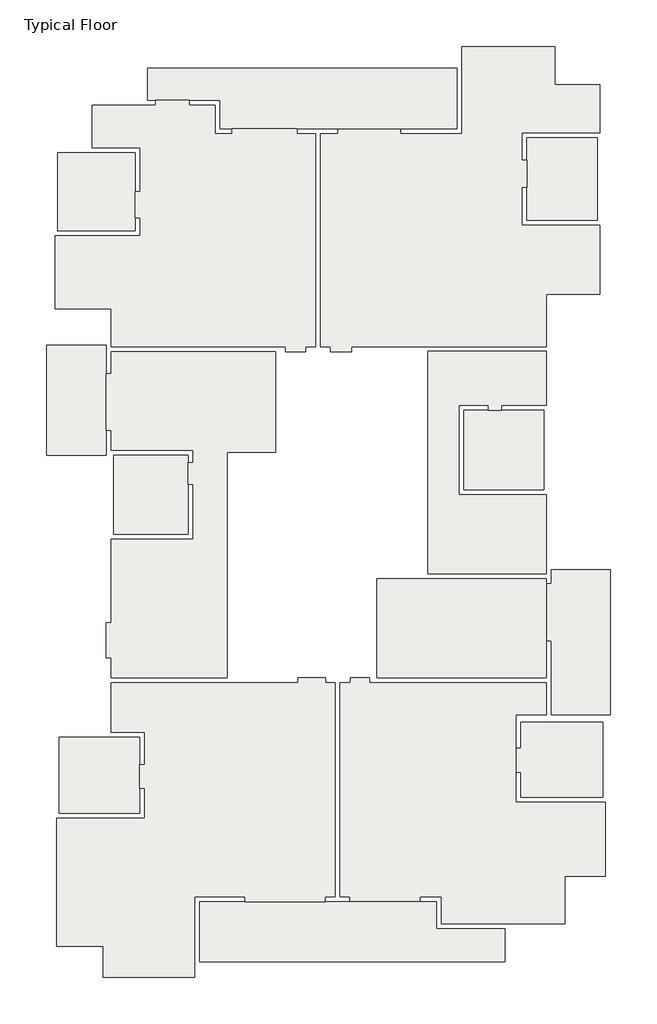
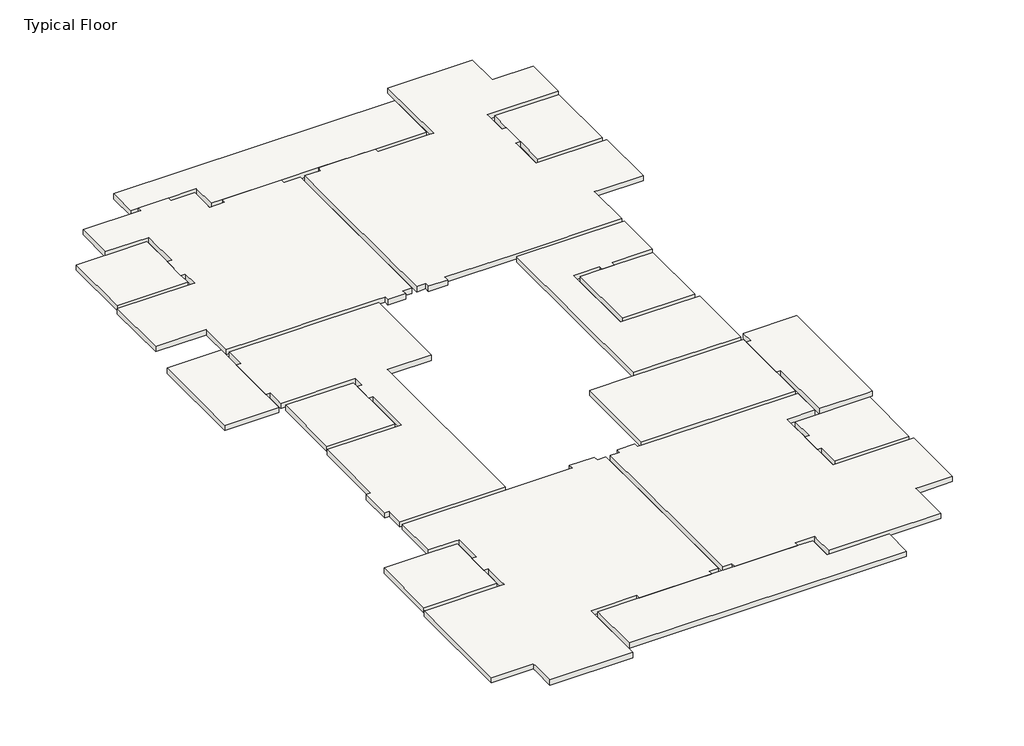
# One storey: 17 slabs.
"""IFC4 building model written with IfcOpenShell, lengths in millimetres."""

from ifc_helpers import new_model, si_unit, frame, origin, place, context, project, spatial, polyline, outline, extrude, faceted_brep, element, save

model = new_model("IFC4")

# Units and contexts
model_context = context("Model", 3, world=origin())
ifc_project = project(units=[si_unit("LENGTHUNIT", "METRE", prefix="MILLI")], contexts=[model_context])

# Site, building, storey
site = spatial("IfcSite", under=ifc_project)
building = spatial("IfcBuilding", under=site)
storey = spatial("IfcBuildingStorey", under=building, Name="Typical Floor", Elevation=3600.0)

# Slabs
placement = place(None, origin())
element("IfcSlab", 1, ObjectType="24", at=placement, inside=storey, context=model_context, shape_type="Brep", body=[
    faceted_brep([(5008.6159742, 7667.3540488, 3360.0), (5008.6159742, 4473.2757833, 3360.0), (1815.6504069, 4473.2757833, 3360.0), (1815.6504069, 7665.1303185, 3360.0), (2790.841428, 7665.1303185, 3360.0), (2790.841428, 7667.3540488, 3360.0), (3310.841428, 7667.3540488, 3360.0), (5008.6159742, 4473.2757833, 3600.0), (5008.6159742, 7667.3540488, 3600.0), (3310.841428, 7667.3540488, 3600.0), (2790.841428, 7667.3540488, 3600.0), (2790.841428, 7665.1303185, 3600.0), (1815.6504069, 7665.1303185, 3600.0), (1815.6504069, 4473.2757833, 3600.0)], [[[0, 1, 2, 3, 4, 5, 6]], [[7, 8, 9, 10, 11, 12, 13]], [[1, 0, 8, 7]], [[2, 1, 7, 13]], [[2, 13, 12, 3]], [[8, 0, 6, 5, 10, 9]], [[11, 4, 3, 12]], [[4, 11, 10, 5]]]),
])
element("IfcSlab", 2, ObjectType="24", at=placement, inside=storey, context=model_context, shape_type="Brep", body=[
    faceted_brep([(5108.6159742, 1118.1901182, 3360.0), (365.5355931, 1118.1901182, 3360.0), (365.5355931, 10002.1270927, 3360.0), (365.5355931, 10011.3193389, 3360.0), (5108.6159742, 10011.3193389, 3360.0), (5108.6159742, 10002.1270927, 3360.0), (5108.6159742, 7867.3540488, 3360.0), (3310.841428, 7867.3540488, 3360.0), (3310.841428, 7667.3540488, 3360.0), (2790.841428, 7667.3540488, 3360.0), (2790.841428, 7865.1303185, 3360.0), (1815.6504069, 7865.1303185, 3360.0), (1615.6504069, 7865.1303185, 3360.0), (1615.6504069, 4473.2757833, 3360.0), (1615.6504069, 4273.2757833, 3360.0), (5108.6159742, 4273.2757833, 3360.0), (365.5355931, 1118.1901182, 3600.0), (1935.6692074, 1118.1901182, 3600.0), (3435.6692074, 1118.1901182, 3600.0), (5108.6159742, 1118.1901182, 3600.0), (5108.6159742, 4273.2757833, 3600.0), (1615.6504069, 4273.2757833, 3600.0), (1615.6504069, 4473.2757833, 3600.0), (1615.6504069, 7865.1303185, 3600.0), (1815.6504069, 7865.1303185, 3600.0), (2790.841428, 7865.1303185, 3600.0), (2790.841428, 7667.3540488, 3600.0), (3310.841428, 7667.3540488, 3600.0), (3310.841428, 7867.3540488, 3600.0), (5108.6159742, 7867.3540488, 3600.0), (5108.6159742, 10011.3193389, 3600.0), (365.5355931, 10011.3193389, 3600.0), (365.5355931, 10002.1270927, 3600.0)], [[[0, 1, 2, 3, 4, 5, 6, 7, 8, 9, 10, 11, 12, 13, 14, 15]], [[16, 17, 18, 19, 20, 21, 22, 23, 24, 25, 26, 27, 28, 29, 30, 31, 32]], [[1, 0, 19, 18, 17, 16]], [[3, 2, 1, 16, 32, 31]], [[4, 3, 31, 30]], [[6, 5, 4, 30, 29]], [[7, 6, 29, 28]], [[7, 28, 27, 8]], [[25, 10, 9, 26]], [[10, 25, 24, 23, 12, 11]], [[12, 23, 22, 21, 14, 13]], [[15, 14, 21, 20]], [[0, 15, 20, 19]], [[9, 8, 27, 26]]]),
])
element("IfcSlab", 3, ObjectType="24", at=placement, inside=storey, context=model_context, shape_type="SweptSolid", body=[
    extrude(outline(polyline([(7152.579426, 18559.8939047), (7152.579426, 15248.7143707), (4325.0704423, 15248.7143707), (4325.0704423, 16574.2647824), (4320.0704423, 16574.2647824), (4320.0704423, 17656.8521012), (4325.0704423, 17656.8521012), (4325.0704423, 18559.8939047), (7152.579426, 18559.8939047)])), frame((0.0, 0.0, 3360.0), z_axis=(0.0, 0.0, 1.0), x_axis=(1.0, 0.0, 0.0)), (0.0, 0.0, 1.0), 240.0),
])
element("IfcSlab", 4, ObjectType="24", at=placement, inside=storey, context=model_context, shape_type="Brep", body=[
    faceted_brep([(-2686.2135861, 10202.1270927, 3360.0), (-2686.2135861, 10002.1270927, 3360.0), (-3531.2135861, 10002.1270927, 3360.0), (-3531.2135861, 10202.1270927, 3360.0), (-3531.8791583, 10202.1270927, 3360.0), (-3936.3283998, 10202.1270927, 3360.0), (-3936.3283998, 18723.1258963, 3360.0), (-3228.5427299, 18723.1258963, 3360.0), (-3228.5427299, 18923.1258963, 3360.0), (-728.3131023, 18923.1258963, 3360.0), (-728.3131023, 18723.1258963, 3360.0), (1532.579426, 18723.1258963, 3360.0), (1732.579426, 18723.1258963, 3360.0), (1732.579426, 22199.8939047, 3360.0), (5452.579426, 22199.8939047, 3360.0), (5452.579426, 20879.8939047, 3360.0), (5452.579426, 20679.8939047, 3360.0), (7252.579426, 20679.8939047, 3360.0), (7252.579426, 18759.8939047, 3360.0), (4325.0704423, 18759.8939047, 3360.0), (4125.0704423, 18759.8939047, 3360.0), (4125.0704423, 17656.8521012, 3360.0), (4320.0704423, 17656.8521012, 3360.0), (4320.0704423, 16574.2647824, 3360.0), (4125.0704423, 16574.2647824, 3360.0), (4125.0704423, 15248.7143707, 3360.0), (4125.0704423, 15048.7143707, 3360.0), (7252.579426, 15048.7143707, 3360.0), (7252.579426, 12288.7143707, 3360.0), (5308.6159742, 12288.7143707, 3360.0), (5108.6159742, 12288.7143707, 3360.0), (5108.6159742, 10202.1270927, 3360.0), (365.5355931, 10202.1270927, 3360.0), (-2686.2135861, 10002.1270927, 3600.0), (-2686.2135861, 10202.1270927, 3600.0), (365.5355931, 10202.1270927, 3600.0), (5108.6159742, 10202.1270927, 3600.0), (5108.6159742, 12288.7143707, 3600.0), (5308.6159742, 12288.7143707, 3600.0), (7252.579426, 12288.7143707, 3600.0), (7252.579426, 15048.7143707, 3600.0), (4125.0704423, 15048.7143707, 3600.0), (4125.0704423, 15248.7143707, 3600.0), (4125.0704423, 16574.2647824, 3600.0), (4320.0704423, 16574.2647824, 3600.0), (4320.0704423, 17656.8521012, 3600.0), (4125.0704423, 17656.8521012, 3600.0), (4125.0704423, 18759.8939047, 3600.0), (4325.0704423, 18759.8939047, 3600.0), (7252.579426, 18759.8939047, 3600.0), (7252.579426, 20679.8939047, 3600.0), (5452.579426, 20679.8939047, 3600.0), (5452.579426, 20879.8939047, 3600.0), (5452.579426, 22199.8939047, 3600.0), (1732.579426, 22199.8939047, 3600.0), (1732.579426, 18723.1258963, 3600.0), (1532.579426, 18723.1258963, 3600.0), (-728.3131023, 18723.1258963, 3600.0), (-728.3131023, 18923.1258963, 3600.0), (-3228.5427299, 18923.1258963, 3600.0), (-3228.5427299, 18723.1258963, 3600.0), (-3936.3283998, 18723.1258963, 3600.0), (-3936.3283998, 16023.1258963, 3600.0), (-3936.3283998, 12523.1258963, 3600.0), (-3936.3283998, 10202.1270927, 3600.0), (-3531.8791583, 10202.1270927, 3600.0), (-3531.2135861, 10202.1270927, 3600.0), (-3531.2135861, 10002.1270927, 3600.0)], [[[0, 1, 2, 3, 4, 5, 6, 7, 8, 9, 10, 11, 12, 13, 14, 15, 16, 17, 18, 19, 20, 21, 22, 23, 24, 25, 26, 27, 28, 29, 30, 31, 32]], [[33, 34, 35, 36, 37, 38, 39, 40, 41, 42, 43, 44, 45, 46, 47, 48, 49, 50, 51, 52, 53, 54, 55, 56, 57, 58, 59, 60, 61, 62, 63, 64, 65, 66, 67]], [[1, 0, 34, 33]], [[2, 1, 33, 67]], [[3, 2, 67, 66]], [[3, 66, 65, 64, 5, 4]], [[6, 5, 64, 63, 62, 61]], [[7, 6, 61, 60]], [[8, 7, 60, 59]], [[9, 8, 59, 58]], [[10, 9, 58, 57]], [[10, 57, 56, 55, 12, 11]], [[13, 12, 55, 54]], [[14, 13, 54, 53]], [[14, 53, 52, 51, 16, 15]], [[17, 16, 51, 50]], [[18, 17, 50, 49]], [[18, 49, 48, 47, 20, 19]], [[21, 20, 47, 46]], [[21, 46, 45, 22]], [[43, 24, 23, 44]], [[24, 43, 42, 41, 26, 25]], [[27, 26, 41, 40]], [[28, 27, 40, 39]], [[28, 39, 38, 37, 30, 29]], [[31, 30, 37, 36]], [[31, 36, 35, 34, 0, 32]], [[23, 22, 45, 44]]]),
])
element("IfcSlab", 5, ObjectType="24", at=placement, inside=storey, context=model_context, shape_type="Brep", body=[
    faceted_brep([(-13057.032521, 19846.7758651, 3360.0), (-10517.8120165, 19846.7758651, 3360.0), (-10517.8120165, 20046.7758651, 3360.0), (-9194.161186, 20046.7758651, 3360.0), (-9194.161186, 19846.7758651, 3360.0), (-8146.2718834, 19846.7758651, 3360.0), (-8146.2718834, 18923.1258963, 3360.0), (-8146.2718834, 18723.1258963, 3360.0), (-7456.8706485, 18723.1258963, 3360.0), (-7456.8706485, 18923.1258963, 3360.0), (-4864.7222926, 18923.1258963, 3360.0), (-4864.7222926, 18723.1258963, 3360.0), (-4136.3283998, 18723.1258963, 3360.0), (-4136.3283998, 10202.1270927, 3360.0), (-4533.8091254, 10202.1270927, 3360.0), (-4533.8091254, 10002.1270927, 3360.0), (-5324.3231159, 10002.1270927, 3360.0), (-5324.3231159, 10202.1270927, 3360.0), (-5726.5468462, 10202.1270927, 3360.0), (-8265.7672932, 10202.1270927, 3360.0), (-9765.7672932, 10202.1270927, 3360.0), (-12310.2559741, 10202.1270927, 3360.0), (-12310.2559741, 11725.7761998, 3360.0), (-12510.2559741, 11725.7761998, 3360.0), (-14552.0616697, 11725.7761998, 3360.0), (-14552.0616697, 14632.6787416, 3360.0), (-11352.0616697, 14632.6787416, 3360.0), (-11152.0616697, 14632.6787416, 3360.0), (-11152.0616697, 15349.6557961, 3360.0), (-11352.0616697, 15349.6557961, 3360.0), (-11352.0616697, 16397.5459604, 3360.0), (-11152.0616697, 16397.5459604, 3360.0), (-11152.0616697, 17945.140638, 3360.0), (-11152.0616697, 18145.140638, 3360.0), (-13057.032521, 18145.140638, 3360.0), (-10517.8120165, 19846.7758651, 3600.0), (-13057.032521, 19846.7758651, 3600.0), (-13057.032521, 18145.140638, 3600.0), (-11152.0616697, 18145.140638, 3600.0), (-11152.0616697, 17945.140638, 3600.0), (-11152.0616697, 16397.5459604, 3600.0), (-11352.0616697, 16397.5459604, 3600.0), (-11352.0616697, 15349.6557961, 3600.0), (-11152.0616697, 15349.6557961, 3600.0), (-11152.0616697, 14632.6787416, 3600.0), (-11352.0616697, 14632.6787416, 3600.0), (-14552.0616697, 14632.6787416, 3600.0), (-14552.0616697, 11725.7761998, 3600.0), (-12510.2559741, 11725.7761998, 3600.0), (-12310.2559741, 11725.7761998, 3600.0), (-12310.2559741, 10202.1270927, 3600.0), (-9765.7672932, 10202.1270927, 3600.0), (-8265.7672932, 10202.1270927, 3600.0), (-5726.5468462, 10202.1270927, 3600.0), (-5324.3231159, 10202.1270927, 3600.0), (-5324.3231159, 10002.1270927, 3600.0), (-4533.8091254, 10002.1270927, 3600.0), (-4533.8091254, 10202.1270927, 3600.0), (-4136.3283998, 10202.1270927, 3600.0), (-4136.3283998, 12523.1258963, 3600.0), (-4136.3283998, 16023.1258963, 3600.0), (-4136.3283998, 18723.1258963, 3600.0), (-4864.7222926, 18723.1258963, 3600.0), (-4864.7222926, 18923.1258963, 3600.0), (-7456.8706485, 18923.1258963, 3600.0), (-7456.8706485, 18723.1258963, 3600.0), (-8146.2718834, 18723.1258963, 3600.0), (-8146.2718834, 18923.1258963, 3600.0), (-8146.2718834, 19846.7758651, 3600.0), (-9194.161186, 19846.7758651, 3600.0), (-9194.161186, 20046.7758651, 3600.0), (-10517.8120165, 20046.7758651, 3600.0)], [[[0, 1, 2, 3, 4, 5, 6, 7, 8, 9, 10, 11, 12, 13, 14, 15, 16, 17, 18, 19, 20, 21, 22, 23, 24, 25, 26, 27, 28, 29, 30, 31, 32, 33, 34]], [[35, 36, 37, 38, 39, 40, 41, 42, 43, 44, 45, 46, 47, 48, 49, 50, 51, 52, 53, 54, 55, 56, 57, 58, 59, 60, 61, 62, 63, 64, 65, 66, 67, 68, 69, 70, 71]], [[1, 0, 36, 35]], [[2, 1, 35, 71]], [[3, 2, 71, 70]], [[4, 3, 70, 69]], [[5, 4, 69, 68]], [[5, 68, 67, 66, 7, 6]], [[8, 7, 66, 65]], [[9, 8, 65, 64]], [[10, 9, 64, 63]], [[11, 10, 63, 62]], [[12, 11, 62, 61]], [[13, 12, 61, 60, 59, 58]], [[14, 13, 58, 57]], [[15, 14, 57, 56]], [[16, 15, 56, 55]], [[17, 16, 55, 54]], [[17, 54, 53, 52, 51, 50, 21, 20, 19, 18]], [[22, 21, 50, 49]], [[22, 49, 48, 47, 24, 23]], [[25, 24, 47, 46]], [[25, 46, 45, 44, 27, 26]], [[28, 27, 44, 43]], [[29, 28, 43, 42]], [[30, 29, 42, 41]], [[31, 30, 41, 40]], [[31, 40, 39, 38, 33, 32]], [[34, 33, 38, 37]], [[0, 34, 37, 36]]]),
])
element("IfcSlab", 6, ObjectType="24", at=placement, inside=storey, context=model_context, shape_type="Brep", body=[
    faceted_brep([(-11352.0616697, 14832.6787416, 3360.0), (-14451.9956956, 14832.6787416, 3360.0), (-14451.9956956, 17945.140638, 3360.0), (-11352.0616697, 17945.140638, 3360.0), (-11352.0616697, 16397.5459604, 3360.0), (-11352.0616697, 15349.6557961, 3360.0), (-14451.9956956, 14832.6787416, 3600.0), (-11352.0616697, 14832.6787416, 3600.0), (-11352.0616697, 15349.6557961, 3600.0), (-11352.0616697, 16397.5459604, 3600.0), (-11352.0616697, 17945.140638, 3600.0), (-13057.032521, 17945.140638, 3600.0), (-13257.032521, 17945.140638, 3600.0), (-14451.9956956, 17945.140638, 3600.0)], [[[0, 1, 2, 3, 4, 5]], [[6, 7, 8, 9, 10, 11, 12, 13]], [[7, 0, 5, 4, 3, 10, 9, 8]], [[1, 0, 7, 6]], [[2, 1, 6, 13]], [[3, 2, 13, 12, 11, 10]]]),
])
element("IfcSlab", 7, ObjectType="24", at=placement, inside=storey, context=model_context, shape_type="Brep", body=[
    faceted_brep([(-5726.5468462, 10002.1270927, 3360.0), (-5726.5468462, 5973.799174, 3360.0), (-7468.2865676, 5973.799174, 3360.0), (-7668.2865676, 5973.799174, 3360.0), (-7668.2865676, -3027.4112609, 3360.0), (-12310.2559741, -3027.4112609, 3360.0), (-12310.2559741, -2234.6718166, 3360.0), (-12510.2559741, -2234.6718166, 3360.0), (-12510.2559741, -828.2926655, 3360.0), (-12310.2559741, -828.2926655, 3360.0), (-12310.2559741, 2508.4085645, 3360.0), (-9219.5123561, 2508.4085645, 3360.0), (-9019.5123561, 2508.4085645, 3360.0), (-9019.5123561, 4705.2999252, 3360.0), (-9219.5123561, 4705.2999252, 3360.0), (-9219.5123561, 5569.3499325, 3360.0), (-9019.5123561, 5569.3499325, 3360.0), (-9019.5123561, 6065.7196834, 3360.0), (-9219.5123561, 6065.7196834, 3360.0), (-12310.2559741, 6065.7196834, 3360.0), (-12310.2559741, 6865.4241392, 3360.0), (-12510.2559741, 6865.4241392, 3360.0), (-12510.2559741, 9117.4688625, 3360.0), (-12310.2559741, 9117.4688625, 3360.0), (-12310.2559741, 10002.1270927, 3360.0), (-5726.5468462, 5973.799174, 3600.0), (-5726.5468462, 10002.1270927, 3600.0), (-8265.7672932, 10002.1270927, 3600.0), (-9765.7672932, 10002.1270927, 3600.0), (-12310.2559741, 10002.1270927, 3600.0), (-12310.2559741, 9117.4688625, 3600.0), (-12510.2559741, 9117.4688625, 3600.0), (-12510.2559741, 6865.4241392, 3600.0), (-12310.2559741, 6865.4241392, 3600.0), (-12310.2559741, 6065.7196834, 3600.0), (-9219.5123561, 6065.7196834, 3600.0), (-9019.5123561, 6065.7196834, 3600.0), (-9019.5123561, 5569.3499325, 3600.0), (-9219.5123561, 5569.3499325, 3600.0), (-9219.5123561, 4705.2999252, 3600.0), (-9019.5123561, 4705.2999252, 3600.0), (-9019.5123561, 2508.4085645, 3600.0), (-9219.5123561, 2508.4085645, 3600.0), (-12310.2559741, 2508.4085645, 3600.0), (-12310.2559741, -828.2926655, 3600.0), (-12510.2559741, -828.2926655, 3600.0), (-12510.2559741, -2234.6718166, 3600.0), (-12310.2559741, -2234.6718166, 3600.0), (-12310.2559741, -3027.4112609, 3600.0), (-7668.2865676, -3027.4112609, 3600.0), (-7668.2865676, 5973.799174, 3600.0), (-7468.2865676, 5973.799174, 3600.0)], [[[0, 1, 2, 3, 4, 5, 6, 7, 8, 9, 10, 11, 12, 13, 14, 15, 16, 17, 18, 19, 20, 21, 22, 23, 24]], [[25, 26, 27, 28, 29, 30, 31, 32, 33, 34, 35, 36, 37, 38, 39, 40, 41, 42, 43, 44, 45, 46, 47, 48, 49, 50, 51]], [[1, 0, 26, 25]], [[1, 25, 51, 50, 3, 2]], [[4, 3, 50, 49]], [[5, 4, 49, 48]], [[6, 5, 48, 47]], [[7, 6, 47, 46]], [[8, 7, 46, 45]], [[9, 8, 45, 44]], [[10, 9, 44, 43]], [[10, 43, 42, 41, 12, 11]], [[13, 12, 41, 40]], [[14, 13, 40, 39]], [[15, 14, 39, 38]], [[16, 15, 38, 37]], [[17, 16, 37, 36]], [[17, 36, 35, 34, 19, 18]], [[20, 19, 34, 33]], [[21, 20, 33, 32]], [[22, 21, 32, 31]], [[23, 22, 31, 30]], [[24, 23, 30, 29]], [[0, 24, 29, 28, 27, 26]]]),
])
element("IfcSlab", 8, ObjectType="24", at=placement, inside=storey, context=model_context, shape_type="Brep", body=[
    faceted_brep([(-9219.5123561, 2708.4085645, 3360.0), (-12210.2559741, 2708.4085645, 3360.0), (-12210.2559741, 5865.7196834, 3360.0), (-9219.5123561, 5865.7196834, 3360.0), (-9219.5123561, 5569.3499325, 3360.0), (-9219.5123561, 4705.2999252, 3360.0), (-12210.2559741, 2708.4085645, 3600.0), (-9219.5123561, 2708.4085645, 3600.0), (-9219.5123561, 4705.2999252, 3600.0), (-9219.5123561, 5569.3499325, 3600.0), (-9219.5123561, 5865.7196834, 3600.0), (-12210.2559741, 5865.7196834, 3600.0)], [[[0, 1, 2, 3, 4, 5]], [[6, 7, 8, 9, 10, 11]], [[7, 0, 5, 4, 3, 10, 9, 8]], [[1, 0, 7, 6]], [[2, 1, 6, 11]], [[3, 2, 11, 10]]]),
])
element("IfcSlab", 9, ObjectType="24", at=placement, inside=storey, context=model_context, shape_type="Brep", body=[
    faceted_brep([(-4837.1456113, -3227.4112609, 3360.0), (-4837.1456113, -3027.4112609, 3360.0), (-3734.1028886, -3027.4112609, 3360.0), (-3734.1028886, -3227.4112609, 3360.0), (-3345.8144093, -3227.4112609, 3360.0), (-3345.8144093, -11796.592326, 3360.0), (-3743.2951349, -11796.592326, 3360.0), (-3743.2951349, -11996.592326, 3360.0), (-6942.1181861, -11996.592326, 3360.0), (-6942.1181861, -11796.592326, 3360.0), (-8771.3292903, -11796.592326, 3360.0), (-8971.3292903, -11796.592326, 3360.0), (-8971.3292903, -15013.7980888, 3360.0), (-12622.7829253, -15013.7980888, 3360.0), (-12622.7829253, -13963.683275, 3360.0), (-12622.7829253, -13763.683275, 3360.0), (-14472.6039184, -13763.683275, 3360.0), (-14472.6039184, -8641.5084419, 3360.0), (-14372.6039184, -8641.5084419, 3360.0), (-10959.0284047, -8641.5084419, 3360.0), (-10959.0284047, -8441.5084419, 3360.0), (-10959.0284047, -7441.5084419, 3360.0), (-11159.0284047, -7441.5084419, 3360.0), (-11159.0284047, -6518.1513745, 3360.0), (-10959.0284047, -6518.1513745, 3360.0), (-10959.0284047, -5203.6927327, 3360.0), (-11159.0284047, -5203.6927327, 3360.0), (-12310.2559741, -5203.6927327, 3360.0), (-12310.2559741, -3227.4112609, 3360.0), (-7668.2865676, -3227.4112609, 3360.0), (-4837.1456113, -3027.4112609, 3600.0), (-4837.1456113, -3227.4112609, 3600.0), (-7668.2865676, -3227.4112609, 3600.0), (-12310.2559741, -3227.4112609, 3600.0), (-12310.2559741, -5203.6927327, 3600.0), (-11159.0284047, -5203.6927327, 3600.0), (-10959.0284047, -5203.6927327, 3600.0), (-10959.0284047, -6518.1513745, 3600.0), (-11159.0284047, -6518.1513745, 3600.0), (-11159.0284047, -7441.5084419, 3600.0), (-10959.0284047, -7441.5084419, 3600.0), (-10959.0284047, -8441.5084419, 3600.0), (-10959.0284047, -8641.5084419, 3600.0), (-14372.6039184, -8641.5084419, 3600.0), (-14472.6039184, -8641.5084419, 3600.0), (-14472.6039184, -13763.683275, 3600.0), (-12622.7829253, -13763.683275, 3600.0), (-12622.7829253, -13963.683275, 3600.0), (-12622.7829253, -15013.7980888, 3600.0), (-8971.3292903, -15013.7980888, 3600.0), (-8971.3292903, -11796.592326, 3600.0), (-8771.3292903, -11796.592326, 3600.0), (-6942.1181861, -11796.592326, 3600.0), (-6942.1181861, -11996.592326, 3600.0), (-3743.2951349, -11996.592326, 3600.0), (-3743.2951349, -11796.592326, 3600.0), (-3345.8144093, -11796.592326, 3600.0), (-3345.8144093, -9275.756314, 3600.0), (-3345.8144093, -5775.756314, 3600.0), (-3345.8144093, -3227.4112609, 3600.0), (-3734.1028886, -3227.4112609, 3600.0), (-3734.1028886, -3027.4112609, 3600.0)], [[[0, 1, 2, 3, 4, 5, 6, 7, 8, 9, 10, 11, 12, 13, 14, 15, 16, 17, 18, 19, 20, 21, 22, 23, 24, 25, 26, 27, 28, 29]], [[30, 31, 32, 33, 34, 35, 36, 37, 38, 39, 40, 41, 42, 43, 44, 45, 46, 47, 48, 49, 50, 51, 52, 53, 54, 55, 56, 57, 58, 59, 60, 61]], [[1, 0, 31, 30]], [[2, 1, 30, 61]], [[3, 2, 61, 60]], [[4, 3, 60, 59]], [[5, 4, 59, 58, 57, 56]], [[6, 5, 56, 55]], [[7, 6, 55, 54]], [[8, 7, 54, 53]], [[9, 8, 53, 52]], [[9, 52, 51, 50, 11, 10]], [[12, 11, 50, 49]], [[13, 12, 49, 48]], [[13, 48, 47, 46, 15, 14]], [[16, 15, 46, 45]], [[17, 16, 45, 44]], [[17, 44, 43, 42, 19, 18]], [[19, 42, 41, 40, 21, 20]], [[22, 21, 40, 39]], [[23, 22, 39, 38]], [[24, 23, 38, 37]], [[25, 24, 37, 36]], [[25, 36, 35, 34, 27, 26]], [[28, 27, 34, 33]], [[28, 33, 32, 31, 0, 29]]]),
])
element("IfcSlab", 10, ObjectType="24", at=placement, inside=storey, context=model_context, shape_type="Brep", body=[
    faceted_brep([(-11159.0284047, -8441.5084419, 3360.0), (-14372.6039184, -8441.5084419, 3360.0), (-14372.6039184, -5402.5799771, 3360.0), (-12310.2559741, -5402.5799771, 3360.0), (-12310.2559741, -5403.6927327, 3360.0), (-11159.0284047, -5403.6927327, 3360.0), (-11159.0284047, -6518.1513745, 3360.0), (-11159.0284047, -7441.5084419, 3360.0), (-14372.6039184, -8441.5084419, 3600.0), (-11159.0284047, -8441.5084419, 3600.0), (-11159.0284047, -7441.5084419, 3600.0), (-11159.0284047, -6518.1513745, 3600.0), (-11159.0284047, -5403.6927327, 3600.0), (-12310.2559741, -5403.6927327, 3600.0), (-12310.2559741, -5402.5799771, 3600.0), (-12510.2559741, -5402.5799771, 3600.0), (-14372.6039184, -5402.5799771, 3600.0)], [[[0, 1, 2, 3, 4, 5, 6, 7]], [[8, 9, 10, 11, 12, 13, 14, 15, 16]], [[9, 0, 7, 6, 5, 12, 11, 10]], [[1, 0, 9, 8]], [[2, 1, 8, 16]], [[2, 16, 15, 14, 3]], [[4, 13, 12, 5]], [[13, 4, 3, 14]]]),
])
element("IfcSlab", 11, ObjectType="24", at=placement, inside=storey, context=model_context, shape_type="Brep", body=[
    faceted_brep([(-1969.2374508, -3027.4112609, 3360.0), (-1969.2374508, -3227.4112609, 3360.0), (-1668.1246952, -3227.4112609, 3360.0), (944.6336071, -3227.4112609, 3360.0), (2444.6336071, -3227.4112609, 3360.0), (5108.6159742, -3227.4112609, 3360.0), (5108.6159742, -4514.2914978, 3360.0), (3886.0795653, -4514.2914978, 3360.0), (3886.0795653, -4814.2914978, 3360.0), (3886.0795653, -5856.32504, 3360.0), (3886.0795653, -6812.2956141, 3360.0), (3886.0795653, -7816.451035, 3360.0), (3886.0795653, -8016.451035, 3360.0), (7454.8049372, -8016.451035, 3360.0), (7454.8049372, -10967.0874585, 3360.0), (6046.2020558, -10967.0874585, 3360.0), (5846.2020558, -10967.0874585, 3360.0), (5846.2020558, -12872.0600908, 3360.0), (898.6742141, -12872.0600908, 3360.0), (898.6742141, -11996.592326, 3360.0), (898.6742141, -11796.592326, 3360.0), (53.0069184, -11796.592326, 3360.0), (53.0069184, -11996.592326, 3360.0), (-2741.3652253, -11996.592326, 3360.0), (-2741.3652253, -11796.592326, 3360.0), (-3145.8144093, -11796.592326, 3360.0), (-3145.8144093, -3227.4112609, 3360.0), (-2732.1747025, -3227.4112609, 3360.0), (-2732.1747025, -3027.4112609, 3360.0), (-1969.2374508, -3227.4112609, 3600.0), (-1969.2374508, -3027.4112609, 3600.0), (-2732.1747025, -3027.4112609, 3600.0), (-2732.1747025, -3227.4112609, 3600.0), (-3145.8144093, -3227.4112609, 3600.0), (-3145.8144093, -5775.756314, 3600.0), (-3145.8144093, -9275.756314, 3600.0), (-3145.8144093, -11796.592326, 3600.0), (-2741.3652253, -11796.592326, 3600.0), (-2741.3652253, -11996.592326, 3600.0), (53.0069184, -11996.592326, 3600.0), (53.0069184, -11796.592326, 3600.0), (898.6742141, -11796.592326, 3600.0), (898.6742141, -11996.592326, 3600.0), (898.6742141, -12872.0600908, 3600.0), (5846.2020558, -12872.0600908, 3600.0), (5846.2020558, -10967.0874585, 3600.0), (6046.2020558, -10967.0874585, 3600.0), (7454.8049372, -10967.0874585, 3600.0), (7454.8049372, -8016.451035, 3600.0), (3886.0795653, -8016.451035, 3600.0), (3886.0795653, -7816.451035, 3600.0), (3886.0795653, -6812.2956141, 3600.0), (3886.0795653, -5856.32504, 3600.0), (3886.0795653, -4814.2914978, 3600.0), (3886.0795653, -4514.2914978, 3600.0), (5108.6159742, -4514.2914978, 3600.0), (5108.6159742, -3227.4112609, 3600.0), (2444.6336071, -3227.4112609, 3600.0), (944.6336071, -3227.4112609, 3600.0), (-1668.1246952, -3227.4112609, 3600.0)], [[[0, 1, 2, 3, 4, 5, 6, 7, 8, 9, 10, 11, 12, 13, 14, 15, 16, 17, 18, 19, 20, 21, 22, 23, 24, 25, 26, 27, 28]], [[29, 30, 31, 32, 33, 34, 35, 36, 37, 38, 39, 40, 41, 42, 43, 44, 45, 46, 47, 48, 49, 50, 51, 52, 53, 54, 55, 56, 57, 58, 59]], [[1, 0, 30, 29]], [[1, 29, 59, 58, 57, 56, 5, 4, 3, 2]], [[6, 5, 56, 55]], [[7, 6, 55, 54]], [[7, 54, 53, 52, 51, 50, 49, 12, 11, 10, 9, 8]], [[13, 12, 49, 48]], [[14, 13, 48, 47]], [[14, 47, 46, 45, 16, 15]], [[17, 16, 45, 44]], [[18, 17, 44, 43]], [[18, 43, 42, 41, 20, 19]], [[21, 20, 41, 40]], [[22, 21, 40, 39]], [[23, 22, 39, 38]], [[24, 23, 38, 37]], [[25, 24, 37, 36]], [[26, 25, 36, 35, 34, 33]], [[27, 26, 33, 32]], [[28, 27, 32, 31]], [[0, 28, 31, 30]]]),
])
element("IfcSlab", 12, ObjectType="24", at=placement, inside=storey, context=model_context, shape_type="SweptSolid", body=[
    extrude(outline(polyline([(7354.8049372, -4814.2914978), (7354.8049372, -7816.451035), (4086.0795653, -7816.451035), (4086.0795653, -6812.2956141), (3886.0795653, -6812.2956141), (3886.0795653, -5856.32504), (4086.0795653, -5856.32504), (4086.0795653, -4814.2914978), (7354.8049372, -4814.2914978)])), frame((0.0, 0.0, 3360.0), z_axis=(0.0, 0.0, 1.0), x_axis=(1.0, 0.0, 0.0)), (0.0, 0.0, 1.0), 240.0),
])
element("IfcSlab", 13, ObjectType="24", at=placement, inside=storey, context=model_context, shape_type="Brep", body=[
    faceted_brep([(5108.6159742, 918.1901182, 3360.0), (5108.6159742, 715.9646069, 3360.0), (5108.6159742, -1563.6550168, 3360.0), (5108.6159742, -3027.4112609, 3360.0), (-1668.1246952, -3027.4112609, 3360.0), (-1668.1246952, 918.1901182, 3360.0), (5108.6159742, 918.1901182, 3600.0), (3435.6692074, 918.1901182, 3600.0), (1935.6692074, 918.1901182, 3600.0), (365.5355931, 918.1901182, 3600.0), (165.5355931, 918.1901182, 3600.0), (-1668.1246952, 918.1901182, 3600.0), (-1668.1246952, -3027.4112609, 3600.0), (944.6336071, -3027.4112609, 3600.0), (2444.6336071, -3027.4112609, 3600.0), (5108.6159742, -3027.4112609, 3600.0), (5108.6159742, -1563.6550168, 3600.0), (5108.6159742, 715.9646069, 3600.0)], [[[0, 1, 2, 3, 4, 5]], [[6, 7, 8, 9, 10, 11, 12, 13, 14, 15, 16, 17]], [[3, 2, 1, 0, 6, 17, 16, 15]], [[4, 3, 15, 14, 13, 12]], [[5, 4, 12, 11]], [[0, 5, 11, 10, 9, 8, 7, 6]]]),
])
element("IfcSlab", 14, ObjectType="24", at=placement, inside=storey, context=model_context, shape_type="Brep", body=[
    faceted_brep([(7654.8049372, 1278.1901182, 3360.0), (7654.8049372, -4514.2914978, 3360.0), (5308.6159742, -4514.2914978, 3360.0), (5308.6159742, -1563.6550168, 3360.0), (5108.6159742, -1563.6550168, 3360.0), (5108.6159742, 715.9646069, 3360.0), (5308.6159742, 715.9646069, 3360.0), (5308.6159742, 1278.1901182, 3360.0), (7654.8049372, -4514.2914978, 3600.0), (7654.8049372, 1278.1901182, 3600.0), (5308.6159742, 1278.1901182, 3600.0), (5308.6159742, 715.9646069, 3600.0), (5108.6159742, 715.9646069, 3600.0), (5108.6159742, -1563.6550168, 3600.0), (5308.6159742, -1563.6550168, 3600.0), (5308.6159742, -4514.2914978, 3600.0), (7354.8049372, -4514.2914978, 3600.0)], [[[0, 1, 2, 3, 4, 5, 6, 7]], [[8, 9, 10, 11, 12, 13, 14, 15, 16]], [[1, 0, 9, 8]], [[2, 1, 8, 16, 15]], [[3, 2, 15, 14]], [[4, 3, 14, 13]], [[5, 4, 13, 12]], [[6, 5, 12, 11]], [[7, 6, 11, 10]], [[0, 7, 10, 9]]]),
])
element("IfcSlab", 15, ObjectType="24", at=placement, inside=storey, context=model_context, shape_type="Brep", body=[
    faceted_brep([(3446.2020558, -14392.0600908, 3360.0), (-8771.3292903, -14392.0600908, 3360.0), (-8771.3292903, -11996.592326, 3360.0), (-6942.1181861, -11996.592326, 3360.0), (-3743.2951349, -11996.592326, 3360.0), (-2741.3652253, -11996.592326, 3360.0), (53.0069184, -11996.592326, 3360.0), (698.6742141, -11996.592326, 3360.0), (698.6742141, -13072.0600908, 3360.0), (898.6742141, -13072.0600908, 3360.0), (3446.2020558, -13072.0600908, 3360.0), (-8771.3292903, -14392.0600908, 3600.0), (3446.2020558, -14392.0600908, 3600.0), (3446.2020558, -13072.0600908, 3600.0), (898.6742141, -13072.0600908, 3600.0), (698.6742141, -13072.0600908, 3600.0), (698.6742141, -11996.592326, 3600.0), (53.0069184, -11996.592326, 3600.0), (-2741.3652253, -11996.592326, 3600.0), (-3743.2951349, -11996.592326, 3600.0), (-6942.1181861, -11996.592326, 3600.0), (-8771.3292903, -11996.592326, 3600.0)], [[[0, 1, 2, 3, 4, 5, 6, 7, 8, 9, 10]], [[11, 12, 13, 14, 15, 16, 17, 18, 19, 20, 21]], [[1, 0, 12, 11]], [[2, 1, 11, 21]], [[3, 2, 21, 20]], [[3, 20, 19, 18, 17, 16, 7, 6, 5, 4]], [[8, 7, 16, 15]], [[8, 15, 14, 13, 10, 9]], [[0, 10, 13, 12]]]),
])
element("IfcSlab", 16, ObjectType="24", at=placement, inside=storey, context=model_context, shape_type="Brep", body=[
    faceted_brep([(-14890.2559741, 5865.7196834, 3360.0), (-14890.2559741, 10265.7196834, 3360.0), (-12510.2559741, 10265.7196834, 3360.0), (-12510.2559741, 9117.4688625, 3360.0), (-12510.2559741, 6865.4241392, 3360.0), (-12510.2559741, 5865.7196834, 3360.0), (-14890.2559741, 10265.7196834, 3600.0), (-14890.2559741, 5865.7196834, 3600.0), (-12510.2559741, 5865.7196834, 3600.0), (-12510.2559741, 6865.4241392, 3600.0), (-12510.2559741, 9117.4688625, 3600.0), (-12510.2559741, 10265.7196834, 3600.0)], [[[0, 1, 2, 3, 4, 5]], [[6, 7, 8, 9, 10, 11]], [[1, 0, 7, 6]], [[2, 1, 6, 11]], [[5, 4, 3, 2, 11, 10, 9, 8]], [[0, 5, 8, 7]]]),
])
element("IfcSlab", 17, ObjectType="24", at=placement, inside=storey, context=model_context, shape_type="Brep", body=[
    faceted_brep([(-10846.2718834, 21326.7758651, 3360.0), (1532.579426, 21326.7758651, 3360.0), (1532.579426, 18923.1258963, 3360.0), (-728.3131023, 18923.1258963, 3360.0), (-3228.5427299, 18923.1258963, 3360.0), (-4864.7222926, 18923.1258963, 3360.0), (-7456.8706485, 18923.1258963, 3360.0), (-7946.2718834, 18923.1258963, 3360.0), (-7946.2718834, 20046.7758651, 3360.0), (-8146.2718834, 20046.7758651, 3360.0), (-9194.161186, 20046.7758651, 3360.0), (-10517.8120165, 20046.7758651, 3360.0), (-10846.2718834, 20046.7758651, 3360.0), (1532.579426, 21326.7758651, 3600.0), (-10846.2718834, 21326.7758651, 3600.0), (-10846.2718834, 20046.7758651, 3600.0), (-10517.8120165, 20046.7758651, 3600.0), (-9194.161186, 20046.7758651, 3600.0), (-8146.2718834, 20046.7758651, 3600.0), (-7946.2718834, 20046.7758651, 3600.0), (-7946.2718834, 18923.1258963, 3600.0), (-7456.8706485, 18923.1258963, 3600.0), (-4864.7222926, 18923.1258963, 3600.0), (-3228.5427299, 18923.1258963, 3600.0), (-728.3131023, 18923.1258963, 3600.0), (1532.579426, 18923.1258963, 3600.0)], [[[0, 1, 2, 3, 4, 5, 6, 7, 8, 9, 10, 11, 12]], [[13, 14, 15, 16, 17, 18, 19, 20, 21, 22, 23, 24, 25]], [[1, 0, 14, 13]], [[2, 1, 13, 25]], [[2, 25, 24, 23, 22, 21, 20, 7, 6, 5, 4, 3]], [[8, 7, 20, 19]], [[8, 19, 18, 17, 16, 15, 12, 11, 10, 9]], [[0, 12, 15, 14]]]),
])

save(model, "model.ifc")

# Revit data of these elements
# Type "24"
#   Function = 0
#   Layers, outside or top first: 24 cm "Concrete" (function 1)
# Element 1 (IfcSlab, "24")
#   Mark = "S1"
#   SOFiSTiK_AMG_Comments = ""
#   Height Offset From Level = 0 cm
#   built-in parameter 1001954 = 1
#   SOFiSTiK_AMG_Scheduled = yes
#   SOFiSTiK_AMG_Adjusted = yes
#   Phase Created = New Construction
#   Materials on its faces: "Concrete"
# Element 2 (IfcSlab, "24")
#   Mark = "S2"
#   SOFiSTiK_AMG_Comments = ""
#   Height Offset From Level = 0 cm
#   built-in parameter 1001954 = 1
#   SOFiSTiK_AMG_Scheduled = yes
#   SOFiSTiK_AMG_Adjusted = yes
#   Phase Created = New Construction
#   Materials on its faces: "Concrete"
# Element 3 (IfcSlab, "24")
#   Mark = "S3"
#   SOFiSTiK_AMG_Comments = ""
#   Height Offset From Level = 0 cm
#   built-in parameter 1001954 = 1
#   SOFiSTiK_AMG_Scheduled = yes
#   SOFiSTiK_AMG_Adjusted = yes
#   Phase Created = New Construction
#   Materials on its faces: "Concrete"
# Element 4 (IfcSlab, "24")
#   Mark = "S4"
#   SOFiSTiK_AMG_Comments = ""
#   built-in parameter 1001955 = 3.14159 (stored number, unit not read)
#   Height Offset From Level = 0 cm
#   built-in parameter 1001954 = 1
#   SOFiSTiK_AMG_Scheduled = yes
#   SOFiSTiK_AMG_Adjusted = yes
#   Phase Created = New Construction
#   Materials on its faces: "Concrete"
# Element 5 (IfcSlab, "24")
#   Mark = "S5"
#   SOFiSTiK_AMG_Comments = ""
#   built-in parameter 1001955 = 1.5708 (stored number, unit not read)
#   Height Offset From Level = 0 cm
#   built-in parameter 1001954 = 1
#   SOFiSTiK_AMG_Scheduled = yes
#   SOFiSTiK_AMG_Adjusted = yes
#   Phase Created = New Construction
#   Materials on its faces: "Concrete"
# Element 6 (IfcSlab, "24")
#   Mark = "S6"
#   SOFiSTiK_AMG_Comments = ""
#   Height Offset From Level = 0 cm
#   built-in parameter 1001954 = 1
#   SOFiSTiK_AMG_Scheduled = yes
#   SOFiSTiK_AMG_Adjusted = yes
#   Phase Created = New Construction
#   Materials on its faces: "Concrete"
# Element 7 (IfcSlab, "24")
#   Mark = "S7"
#   SOFiSTiK_AMG_Comments = ""
#   Height Offset From Level = 0 cm
#   built-in parameter 1001954 = 1
#   SOFiSTiK_AMG_Scheduled = yes
#   SOFiSTiK_AMG_Adjusted = yes
#   Phase Created = New Construction
#   Materials on its faces: "Concrete"
# Element 8 (IfcSlab, "24")
#   Mark = "S8"
#   SOFiSTiK_AMG_Comments = ""
#   Height Offset From Level = 0 cm
#   built-in parameter 1001954 = 1
#   SOFiSTiK_AMG_Scheduled = yes
#   SOFiSTiK_AMG_Adjusted = yes
#   Phase Created = New Construction
#   Materials on its faces: "Concrete"
# Element 9 (IfcSlab, "24")
#   Mark = "S9"
#   SOFiSTiK_AMG_Comments = ""
#   Height Offset From Level = 0 cm
#   built-in parameter 1001954 = 1
#   SOFiSTiK_AMG_Scheduled = yes
#   SOFiSTiK_AMG_Adjusted = yes
#   Phase Created = New Construction
#   Materials on its faces: "Concrete"
# Element 10 (IfcSlab, "24")
#   Mark = "S10"
#   SOFiSTiK_AMG_Comments = ""
#   Height Offset From Level = 0 cm
#   built-in parameter 1001954 = 1
#   SOFiSTiK_AMG_Scheduled = yes
#   SOFiSTiK_AMG_Adjusted = yes
#   Phase Created = New Construction
#   Materials on its faces: "Concrete"
# Element 11 (IfcSlab, "24")
#   Mark = "S11"
#   SOFiSTiK_AMG_Comments = ""
#   Height Offset From Level = 0 cm
#   built-in parameter 1001954 = 1
#   SOFiSTiK_AMG_Scheduled = yes
#   SOFiSTiK_AMG_Adjusted = yes
#   Phase Created = New Construction
#   Materials on its faces: "Concrete"
# Element 12 (IfcSlab, "24")
#   Mark = "S12"
#   SOFiSTiK_AMG_Comments = ""
#   Height Offset From Level = 0 cm
#   built-in parameter 1001954 = 1
#   SOFiSTiK_AMG_Scheduled = yes
#   SOFiSTiK_AMG_Adjusted = yes
#   Phase Created = New Construction
#   Materials on its faces: "Concrete"
# Element 13 (IfcSlab, "24")
#   Mark = "S13"
#   SOFiSTiK_AMG_Comments = ""
#   Height Offset From Level = 0 cm
#   built-in parameter 1001954 = 1
#   SOFiSTiK_AMG_Scheduled = yes
#   SOFiSTiK_AMG_Adjusted = yes
#   Phase Created = New Construction
#   Materials on its faces: "Concrete"
# Element 14 (IfcSlab, "24")
#   Mark = "S14"
#   SOFiSTiK_AMG_Comments = ""
#   Height Offset From Level = 0 cm
#   built-in parameter 1001954 = 1
#   SOFiSTiK_AMG_Scheduled = yes
#   SOFiSTiK_AMG_Adjusted = yes
#   Phase Created = New Construction
#   Materials on its faces: "Concrete"
# Element 15 (IfcSlab, "24")
#   Mark = "S15"
#   SOFiSTiK_AMG_Comments = ""
#   built-in parameter 1001955 = -1.5708 (stored number, unit not read)
#   Height Offset From Level = 0 cm
#   built-in parameter 1001954 = 1
#   SOFiSTiK_AMG_Scheduled = yes
#   SOFiSTiK_AMG_Adjusted = yes
#   Phase Created = New Construction
#   Materials on its faces: "Concrete"
# Element 16 (IfcSlab, "24")
#   Mark = "S16"
#   SOFiSTiK_AMG_Comments = ""
#   built-in parameter 1001955 = 3.14159 (stored number, unit not read)
#   Height Offset From Level = 0 cm
#   built-in parameter 1001954 = 1
#   SOFiSTiK_AMG_Scheduled = yes
#   SOFiSTiK_AMG_Adjusted = yes
#   Phase Created = New Construction
#   Materials on its faces: "Concrete"
# Element 17 (IfcSlab, "24")
#   Mark = "S17"
#   SOFiSTiK_AMG_Comments = ""
#   built-in parameter 1001955 = 1.5708 (stored number, unit not read)
#   Height Offset From Level = 0 cm
#   built-in parameter 1001954 = 1
#   SOFiSTiK_AMG_Scheduled = yes
#   SOFiSTiK_AMG_Adjusted = yes
#   Phase Created = New Construction
#   Materials on its faces: "Concrete"
# Materials
#   "Concrete": class "Concrete", colour RGB 192 192 192, transparency 0, Keynote = "01000", Description = "Cast-in-place concrete", Cost = 0
